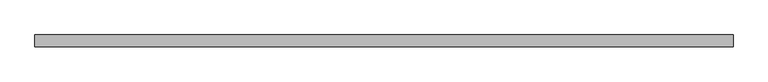
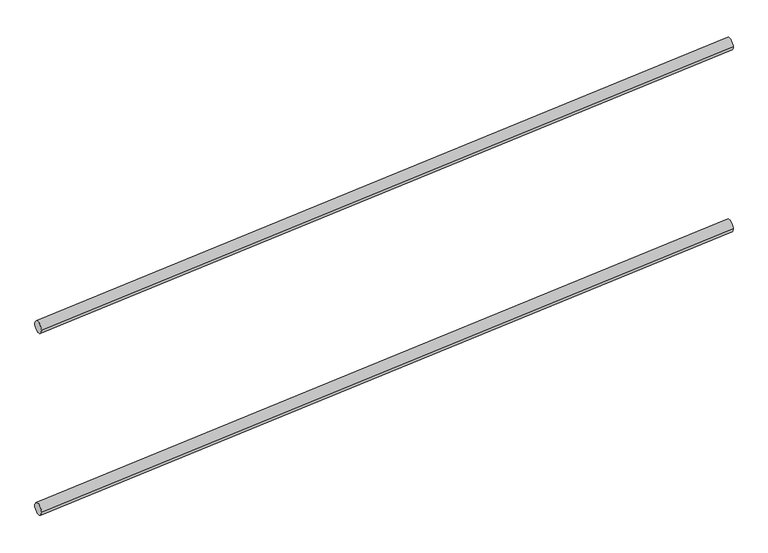
"""IFC4 building model written with IfcOpenShell, lengths in millimetres: railing geometry."""

from ifc_helpers import new_model, si_unit, frame, origin, place, context, project, spatial, ellipse_curve, source, transform, mapped, element, save
from ifc_brep_helpers import plane_surface, cylinder_surface, advanced_brep


def railing_9620f236(model_context):
    return source(origin(), model_context, "Body", "AdvancedBrep", [
        advanced_brep(
        [(-2175.3, 21567.264479, 584.9480068), (-2175.3, 21537.264479, 584.9480068), (-375.3, 21567.264479, 734.9480068), (-375.3, 21537.264479, 734.9480068)],
        [
            (0, 1, ellipse_curve(frame((-2175.3, 21552.264479, 584.9480068), z_axis=(-1.0, 0.0, 0.0), x_axis=(0.0, 0.0, -0.9999999999999999)), 15.0519932, 15.0)),
            (1, 0, ellipse_curve(frame((-2175.3, 21552.264479, 584.9480068), z_axis=(-1.0, 0.0, 0.0), x_axis=(0.0, 0.0, -0.9999999999999999)), 15.0519932, 15.0)),
            (2, 3, ellipse_curve(frame((-375.3, 21552.264479, 734.9480068), z_axis=(1.0, 0.0, 0.0), x_axis=(0.0, 0.0, -0.9999999999999999)), 15.0519932, 15.0)),
            (3, 2, ellipse_curve(frame((-375.3, 21552.264479, 734.9480068), z_axis=(1.0, 0.0, 0.0), x_axis=(0.0, 0.0, -0.9999999999999999)), 15.0519932, 15.0)),
            (0, 2),
            (3, 1),
        ],
        [
            plane_surface(frame((-2175.3, 21552.264479, 600.0), z_axis=(-1.0, 0.0, 0.0), x_axis=(0.0, 1.0, 0.0))),
            plane_surface(frame((-375.3, 21552.264479, 750.0), z_axis=(1.0, 0.0, 0.0), x_axis=(0.0, 1.0, 0.0))),
            cylinder_surface(frame((-2174.0543178, 21552.264479, 585.0518136), z_axis=(-0.9965457582448797, 0.0, -0.08304547985373997), x_axis=(0.0, -1.0, 0.0)), 15.0),
        ],
        [
            (0, [[1, 2]]),
            (1, [[3, 4]]),
            (2, [[-1, 5, -4, 6]]),
            (2, [[-2, -6, -3, -5]]),
        ],
    ),
        advanced_brep(
        [(-2175.3, 21567.264479, 1084.9480068), (-2175.3, 21537.264479, 1084.9480068), (-375.3, 21567.264479, 1234.9480068), (-375.3, 21537.264479, 1234.9480068)],
        [
            (0, 1, ellipse_curve(frame((-2175.3, 21552.264479, 1084.9480068), z_axis=(-1.0, 0.0, 0.0), x_axis=(0.0, 0.0, -0.9999999999999999)), 15.0519932, 15.0)),
            (1, 0, ellipse_curve(frame((-2175.3, 21552.264479, 1084.9480068), z_axis=(-1.0, 0.0, 0.0), x_axis=(0.0, 0.0, -0.9999999999999999)), 15.0519932, 15.0)),
            (2, 3, ellipse_curve(frame((-375.3, 21552.264479, 1234.9480068), z_axis=(1.0, 0.0, 0.0), x_axis=(0.0, 0.0, -0.9999999999999999)), 15.0519932, 15.0)),
            (3, 2, ellipse_curve(frame((-375.3, 21552.264479, 1234.9480068), z_axis=(1.0, 0.0, 0.0), x_axis=(0.0, 0.0, -0.9999999999999999)), 15.0519932, 15.0)),
            (0, 2),
            (3, 1),
        ],
        [
            plane_surface(frame((-2175.3, 21552.264479, 1100.0), z_axis=(-1.0, 0.0, 0.0), x_axis=(0.0, 1.0, 0.0))),
            plane_surface(frame((-375.3, 21552.264479, 1250.0), z_axis=(1.0, 0.0, 0.0), x_axis=(0.0, 1.0, 0.0))),
            cylinder_surface(frame((-2174.0543178, 21552.264479, 1085.0518136), z_axis=(-0.9965457582448797, 0.0, -0.08304547985373997), x_axis=(0.0, -1.0, 0.0)), 15.0),
        ],
        [
            (0, [[1, 2]]),
            (1, [[3, 4]]),
            (2, [[-1, 5, -4, 6]]),
            (2, [[-2, -6, -3, -5]]),
        ],
    ),
    ])


if __name__ == "__main__":
    model = new_model("IFC4")
    model_context = context("Model", 3, world=origin())
    ifc_project = project(units=[si_unit("LENGTHUNIT", "METRE", prefix="MILLI")], contexts=[model_context])
    site = spatial("IfcSite", under=ifc_project)
    building = spatial("IfcBuilding", under=site)
    placement = place(None, origin())
    railing_shape = railing_9620f236(model_context)
    element("IfcRailing", 1, at=placement, inside=building, context=model_context, shape_type="MappedRepresentation", body=[
        mapped(railing_shape, transform((0.0, 0.0, 0.0), x_axis=(1.0, 0.0, 0.0), y_axis=(0.0, 1.0, 0.0), z_axis=(0.0, 0.0, 1.0))),
    ])
    save(model, "model.ifc")
